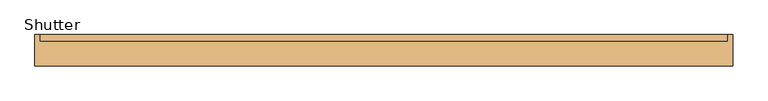
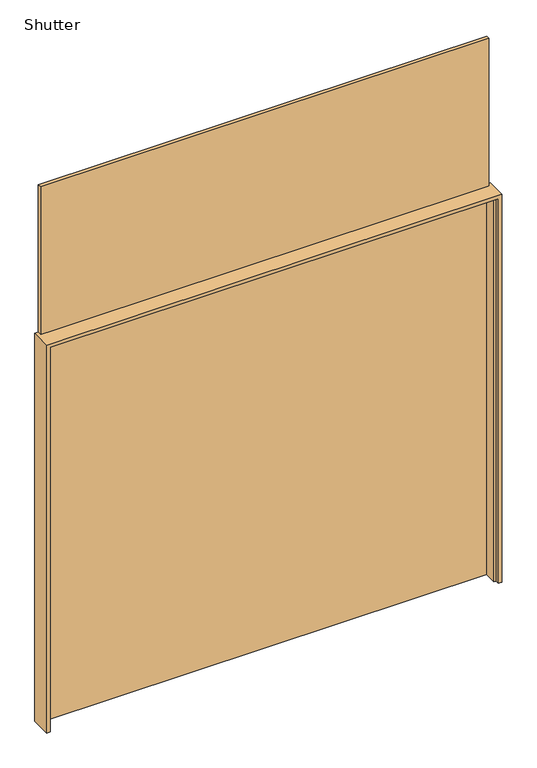
"""IFC4 building model written with IfcOpenShell, lengths in millimetres: door geometry, Shutter : H_DR_AR_B12_Roll up Door_Steel_Manual_W4000xH5000_SRD1."""

from ifc_helpers import new_model, si_unit, origin, origin_with_axes, place, context, project, spatial, polyline, outline, extrude, faceted_brep, source, transform, mapped, element, save


def shutter_8409c925(model_context):
    return source(origin(), model_context, "Body", "SolidModel", [
        extrude(outline(polyline([(1970.0, 90.0), (1970.0, 55.0), (-1970.0, 55.0), (-1970.0, 90.0), (1970.0, 90.0)])), origin_with_axes(), (0.0, 0.0, 1.0), 4970.0),
        faceted_brep([(1970.0, 90.0, 0.0), (2000.0, 90.0, 0.0), (2000.0, -90.0, 0.0), (1970.0, -90.0, 0.0), (1970.0, -55.0, 0.0), (1950.0, -55.0, 0.0), (1950.0, 55.0, 0.0), (1970.0, 55.0, 0.0), (1970.0, 90.0, 3570.0), (-1970.0, 90.0, 3570.0), (-1970.0, 90.0, 0.0), (-2000.0, 90.0, 0.0), (-2000.0, 90.0, 3600.0), (2000.0, 90.0, 3600.0), (2000.0, -90.0, 3600.0), (-2000.0, -90.0, 3600.0), (-2000.0, -90.0, 0.0), (-1970.0, -90.0, 0.0), (-1970.0, -90.0, 3570.0), (1970.0, -90.0, 3570.0), (1970.0, -55.0, 3570.0), (-1970.0, -55.0, 3570.0), (-1970.0, -55.0, 0.0), (-1950.0, -55.0, 0.0), (-1950.0, -55.0, 3550.0), (1950.0, -55.0, 3550.0), (1950.0, 55.0, 3550.0), (-1950.0, 55.0, 3550.0), (-1950.0, 55.0, 0.0), (-1970.0, 55.0, 0.0), (-1970.0, 55.0, 3570.0), (1970.0, 55.0, 3570.0)], [[[0, 1, 2, 3, 4, 5, 6, 7]], [[1, 0, 8, 9, 10, 11, 12, 13]], [[2, 1, 13, 14]], [[3, 2, 14, 15, 16, 17, 18, 19]], [[4, 3, 19, 20]], [[5, 4, 20, 21, 22, 23, 24, 25]], [[6, 5, 25, 26]], [[7, 6, 26, 27, 28, 29, 30, 31]], [[0, 7, 31, 8]], [[9, 30, 29, 10]], [[10, 29, 28, 23, 22, 17, 16, 11]], [[15, 12, 11, 16]], [[21, 18, 17, 22]], [[27, 24, 23, 28]], [[8, 31, 30, 9]], [[14, 13, 12, 15]], [[20, 19, 18, 21]], [[26, 25, 24, 27]]]),
    ])


if __name__ == "__main__":
    model = new_model("IFC4")
    model_context = context("Model", 3, world=origin())
    ifc_project = project(units=[si_unit("LENGTHUNIT", "METRE", prefix="MILLI")], contexts=[model_context])
    site = spatial("IfcSite", under=ifc_project)
    building = spatial("IfcBuilding", under=site)
    placement = place(None, origin())
    shutter_shape = shutter_8409c925(model_context)
    element("IfcDoor", 1, ObjectType="Shutter : H_DR_AR_B12_Roll up Door_Steel_Manual_W4000xH5000_SRD1", at=placement, inside=building, context=model_context, shape_type="MappedRepresentation", body=[
        mapped(shutter_shape, transform((0.0, 0.0, 0.0), x_axis=(1.0, 0.0, 0.0), y_axis=(0.0, 1.0, 0.0), z_axis=(0.0, 0.0, 1.0))),
    ])
    save(model, "model.ifc")

# Revit data of these elements
# Type "Shutter : H_DR_AR_B12_Roll up Door_Steel_Manual_W4000xH5000_SRD1"
#   Type Mark = "431"
#   Analytic Construction = "<None>"
#   프레임 투영 외부. = 25 mm
#   프레임 투영 내부. = 25 mm
#   프레임 폭 = 75 mm
#   Height = 5000 mm
#   Width = 4000 mm
#   Define Thermal Properties by = 1
#   문 패널 = none
#   문 프레임 = none
#   Function = (empty or 0)
#   Wall Closure = (empty or 0)
